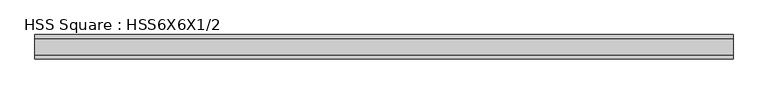
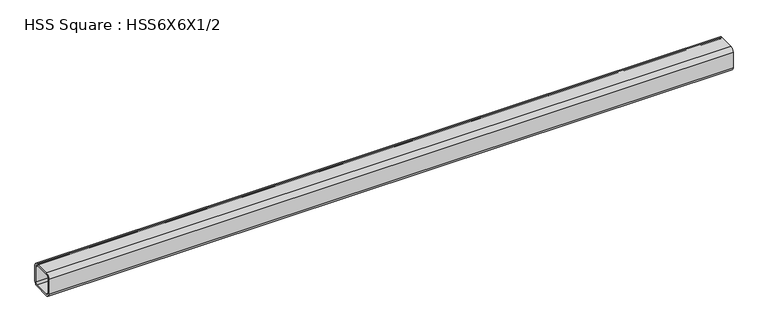
"""IFC4 building model written with IfcOpenShell, lengths in millimetres: member geometry, HSS Square : HSS6X6X1/2."""

from ifc_helpers import new_model, si_unit, point, frame, frame_2d, origin, place, context, project, spatial, polyline, circle_curve, trimmed, segment, composite_curve, outline, extrude, source, transform, mapped, element, save


def hss_square_hss6x6x1_2_596f4375(model_context):
    return source(origin(), model_context, "Body", "SweptSolid", [
        extrude(outline(composite_curve([segment(polyline([(76.2, 50.8), (76.2, -50.8)]), True, "CONTINUOUS"), segment(trimmed(circle_curve(frame_2d((50.8, -50.8)), 25.4), [point((76.2, -50.8))], [point((50.8, -76.2))], False, "CARTESIAN"), True, "CONTINUOUS"), segment(polyline([(50.8, -76.2), (-50.8, -76.2)]), True, "CONTINUOUS"), segment(trimmed(circle_curve(frame_2d((-50.8, -50.8)), 25.4), [point((-50.8, -76.2))], [point((-76.2, -50.8))], False, "CARTESIAN"), True, "CONTINUOUS"), segment(polyline([(-76.2, -50.8), (-76.2, 50.8)]), True, "CONTINUOUS"), segment(trimmed(circle_curve(frame_2d((-50.8, 50.8)), 25.4), [point((-76.2, 50.8))], [point((-50.8, 76.2))], False, "CARTESIAN"), True, "CONTINUOUS"), segment(polyline([(-50.8, 76.2), (50.8, 76.2)]), True, "CONTINUOUS"), segment(trimmed(circle_curve(frame_2d((50.8, 50.8)), 25.4), [point((50.8, 76.2))], [point((76.2, 50.8))], False, "CARTESIAN"), True, "CONTINUOUS")], self_intersect=False), holes=[composite_curve([segment(trimmed(circle_curve(frame_2d((-50.8, 50.8)), 12.7), [point((-50.8, 63.5))], [point((-63.5, 50.8))], True, "CARTESIAN"), True, "CONTINUOUS"), segment(polyline([(-63.5, 50.8), (-63.5, -50.8)]), True, "CONTINUOUS"), segment(trimmed(circle_curve(frame_2d((-50.8, -50.8)), 12.7), [point((-63.5, -50.8))], [point((-50.8, -63.5))], True, "CARTESIAN"), True, "CONTINUOUS"), segment(polyline([(-50.8, -63.5), (50.8, -63.5)]), True, "CONTINUOUS"), segment(trimmed(circle_curve(frame_2d((50.8, -50.8)), 12.7), [point((50.8, -63.5))], [point((63.5, -50.8))], True, "CARTESIAN"), True, "CONTINUOUS"), segment(polyline([(63.5, -50.8), (63.5, 50.8)]), True, "CONTINUOUS"), segment(trimmed(circle_curve(frame_2d((50.8, 50.8)), 12.7), [point((63.5, 50.8))], [point((50.8, 63.5))], True, "CARTESIAN"), True, "CONTINUOUS"), segment(polyline([(50.8, 63.5), (-50.8, 63.5)]), True, "CONTINUOUS")], self_intersect=False)]), frame((-2175.5187939, 0.0, 0.0), z_axis=(1.0, 0.0, 0.0), x_axis=(0.0, 1.0, 0.0)), (0.0, 0.0, 1.0), 4351.0375878),
    ])


if __name__ == "__main__":
    model = new_model("IFC4")
    model_context = context("Model", 3, world=origin())
    ifc_project = project(units=[si_unit("LENGTHUNIT", "METRE", prefix="MILLI")], contexts=[model_context])
    site = spatial("IfcSite", under=ifc_project)
    building = spatial("IfcBuilding", under=site)
    placement = place(None, origin())
    hss_square_hss6x6x1_2_shape = hss_square_hss6x6x1_2_596f4375(model_context)
    element("IfcMember", 1, ObjectType="HSS Square : HSS6X6X1/2", at=placement, inside=building, context=model_context, shape_type="MappedRepresentation", body=[
        mapped(hss_square_hss6x6x1_2_shape, transform((0.0, 0.0, 0.0), x_axis=(1.0, 0.0, 0.0), y_axis=(0.0, 1.0, 0.0), z_axis=(0.0, 0.0, 1.0))),
    ])
    save(model, "model.ifc")

# Revit data of these elements
# Type "HSS Square : HSS6X6X1/2"
#   Section Name Key = "HSS 6X6X1/2"
#   Assembly Code = "B10"
#   Width = 6.000"
#   Wall Nominal Thickness = 0.500"
#   Wall Design Thickness = 0.465"
#   Torsional Moment of Inertia = 81.10 in⁴
#   Torsional Modulus = 28.10 in³
#   Section Area = 9.74 in²
#   Plastic Modulus weak axis = 19.80 in³
#   Plastic Modulus strong axis = 19.80 in³
#   Outer Fillet = 1.000"
#   Nominal Weight = 35.24 lbf/ft
#   Moment of Inertia weak axis = 48.30 in⁴
#   Moment of Inertia strong axis = 48.30 in⁴
#   Inner Fillet = 0.500"
#   Height = 6.000"
#   Elastic Modulus weak axis = 16.10 in³
#   Elastic Modulus strong axis = 16.10 in³
#   Centroid Vertical = 3.000"
#   Centroid Horizontal = 3.000"
#   Length [instance default] = 5' - 0"
#   Structural Material [instance default] = Steel ASTM A500, Grade B, Rectangular and Square
#   Principal Axes Angle = 0
# Element 1 (IfcMember, "HSS Square : HSS6X6X1/2")
#   Structural Material = Steel ASTM A36
#   Materials on its faces: "Steel ASTM A36"
# Materials
#   "Steel ASTM A500, Grade B, Rectangular and Square": class "Metal", colour RGB 199 199 199, transparency 0, Description = "Carbon steel", Cost = 0
#   "Steel ASTM A36": class "Metal", colour RGB 199 199 199, transparency 0, Description = "Structural steel, ASTM A36 Grade B, mill finish", Cost = 0
